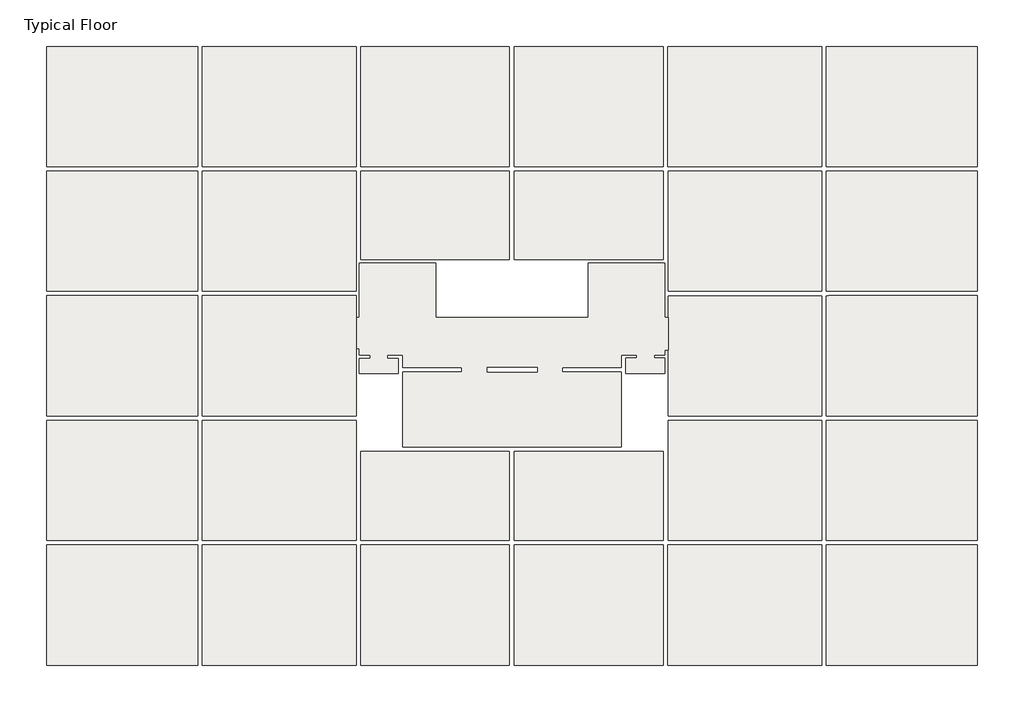
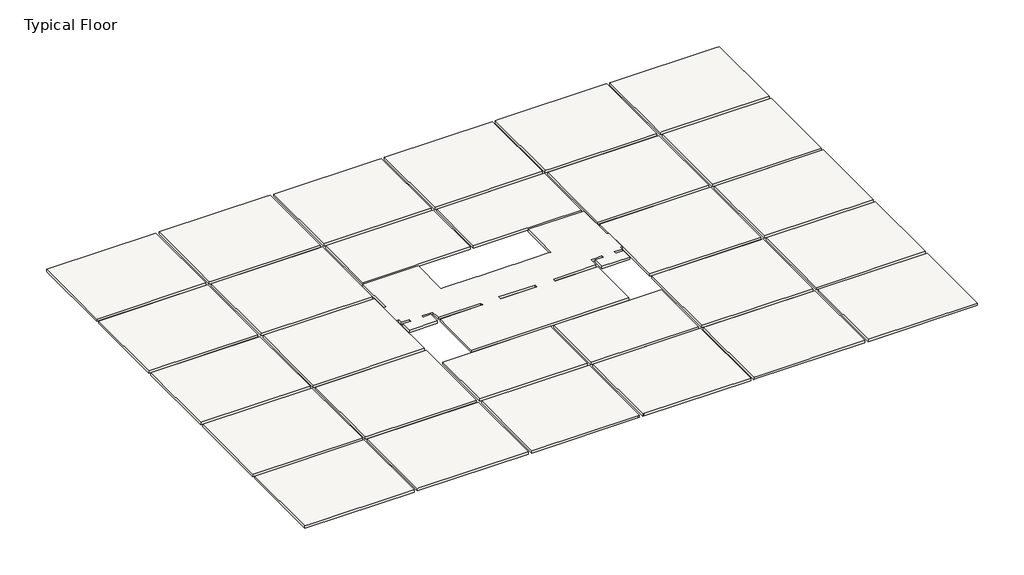
# One storey: 29 slabs.
"""IFC4 building model written with IfcOpenShell, lengths in millimetres."""

from ifc_helpers import new_model, si_unit, origin, place, context, project, spatial, faceted_brep, element, save

model = new_model("IFC4")

# Units and contexts
model_context = context("Model", 3, world=origin())
ifc_project = project(units=[si_unit("LENGTHUNIT", "METRE", prefix="MILLI")], contexts=[model_context])

# Site, building, storey
site = spatial("IfcSite", under=ifc_project)
building = spatial("IfcBuilding", under=site)
storey = spatial("IfcBuildingStorey", under=building, Name="Typical Floor", Elevation=3080.0)

# Slabs
placement = place(None, origin())
element("IfcSlab", 1, ObjectType="22", at=placement, inside=storey, context=model_context, shape_type="Brep", body=[
    faceted_brep([(-16600.7819865, 24775.4190544, 2860.0), (-16600.7819865, 17073.0342824, 2860.0), (-26299.1167382, 17073.0342824, 2860.0), (-26299.1167382, 24775.4190544, 2860.0), (-16600.7819865, 24775.4190544, 3080.0), (-16750.7819865, 24775.4190544, 3080.0), (-25999.1167382, 24775.4190544, 3080.0), (-26299.1167382, 24775.4190544, 3080.0), (-26299.1167382, 17073.0342824, 3080.0), (-16750.7819865, 17073.0342824, 3080.0), (-16600.7819865, 17073.0342824, 3080.0)], [[[0, 1, 2, 3]], [[4, 5, 6, 7, 8, 9, 10]], [[1, 0, 4, 10]], [[2, 1, 10, 9, 8]], [[3, 2, 8, 7]], [[0, 3, 7, 6, 5, 4]]]),
])
element("IfcSlab", 2, ObjectType="22", at=placement, inside=storey, context=model_context, shape_type="Brep", body=[
    faceted_brep([(-6447.328783, 24775.4190544, 2860.0), (-6447.328783, 17073.0342824, 2860.0), (-16300.7819865, 17073.0342824, 2860.0), (-16300.7819865, 24775.4190544, 2860.0), (-6447.328783, 24775.4190544, 3080.0), (-6747.328783, 24775.4190544, 3080.0), (-16150.7819865, 24775.4190544, 3080.0), (-16300.7819865, 24775.4190544, 3080.0), (-16300.7819865, 17073.0342824, 3080.0), (-16150.7819865, 17073.0342824, 3080.0), (-6747.328783, 17073.0342824, 3080.0), (-6447.328783, 17073.0342824, 3080.0)], [[[0, 1, 2, 3]], [[4, 5, 6, 7, 8, 9, 10, 11]], [[1, 0, 4, 11]], [[2, 1, 11, 10, 9, 8]], [[3, 2, 8, 7]], [[0, 3, 7, 6, 5, 4]]]),
])
element("IfcSlab", 3, ObjectType="22", at=placement, inside=storey, context=model_context, shape_type="Brep", body=[
    faceted_brep([(-6447.328783, 16773.0342824, 2860.0), (-6447.328783, 9078.7943074, 2860.0), (-16300.7819865, 9078.7943074, 2860.0), (-16300.7819865, 16773.0342824, 2860.0), (-6447.328783, 16773.0342824, 3080.0), (-6747.328783, 16773.0342824, 3080.0), (-16150.7819865, 16773.0342824, 3080.0), (-16300.7819865, 16773.0342824, 3080.0), (-16300.7819865, 9078.7943074, 3080.0), (-16150.7819865, 9078.7943074, 3080.0), (-6447.328783, 9078.7943074, 3080.0), (-6447.328783, 11089.5351037, 3080.0)], [[[0, 1, 2, 3]], [[4, 5, 6, 7, 8, 9, 10, 11]], [[1, 0, 4, 11, 10]], [[2, 1, 10, 9, 8]], [[3, 2, 8, 7]], [[0, 3, 7, 6, 5, 4]]]),
])
element("IfcSlab", 4, ObjectType="22", at=placement, inside=storey, context=model_context, shape_type="Brep", body=[
    faceted_brep([(-16600.7819865, 16773.0342824, 2860.0), (-16600.7819865, 9078.7943074, 2860.0), (-26299.1167382, 9078.7943074, 2860.0), (-26299.1167382, 16773.0342824, 2860.0), (-16600.7819865, 16773.0342824, 3080.0), (-16750.7819865, 16773.0342824, 3080.0), (-26299.1167382, 16773.0342824, 3080.0), (-26299.1167382, 9078.7943074, 3080.0), (-16750.7819865, 9078.7943074, 3080.0), (-16600.7819865, 9078.7943074, 3080.0)], [[[0, 1, 2, 3]], [[4, 5, 6, 7, 8, 9]], [[1, 0, 4, 9]], [[2, 1, 9, 8, 7]], [[3, 2, 7, 6]], [[0, 3, 6, 5, 4]]]),
])
element("IfcSlab", 5, ObjectType="22", at=placement, inside=storey, context=model_context, shape_type="Brep", body=[
    faceted_brep([(-16600.7819865, 8778.7943074, 2860.0), (-16600.7819865, 1074.102585, 2860.0), (-26299.1167382, 1074.102585, 2860.0), (-26299.1167382, 8778.7943074, 2860.0), (-16600.7819865, 8778.7943074, 3080.0), (-16750.7819865, 8778.7943074, 3080.0), (-26299.1167382, 8778.7943074, 3080.0), (-26299.1167382, 1074.102585, 3080.0), (-16750.7819865, 1074.102585, 3080.0), (-16600.7819865, 1074.102585, 3080.0)], [[[0, 1, 2, 3]], [[4, 5, 6, 7, 8, 9]], [[1, 0, 4, 9]], [[2, 1, 9, 8, 7]], [[3, 2, 7, 6]], [[0, 3, 6, 5, 4]]]),
])
element("IfcSlab", 6, ObjectType="22", at=placement, inside=storey, context=model_context, shape_type="Brep", body=[
    faceted_brep([(-16600.7819865, 774.102585, 2860.0), (-16600.7819865, -6920.4648963, 2860.0), (-26299.1167382, -6920.4648963, 2860.0), (-26299.1167382, 774.102585, 2860.0), (-16600.7819865, 774.102585, 3080.0), (-16750.7819865, 774.102585, 3080.0), (-26299.1167382, 774.102585, 3080.0), (-26299.1167382, -6920.4648963, 3080.0), (-16750.7819865, -6920.4648963, 3080.0), (-16600.7819865, -6920.4648963, 3080.0)], [[[0, 1, 2, 3]], [[4, 5, 6, 7, 8, 9]], [[1, 0, 4, 9]], [[2, 1, 9, 8, 7]], [[3, 2, 7, 6]], [[0, 3, 6, 5, 4]]]),
])
element("IfcSlab", 7, ObjectType="22", at=placement, inside=storey, context=model_context, shape_type="Brep", body=[
    faceted_brep([(-6447.328783, 774.102585, 2860.0), (-6447.328783, -6920.4648963, 2860.0), (-16300.7819865, -6920.4648963, 2860.0), (-16300.7819865, 774.102585, 2860.0), (-6447.328783, 774.102585, 3080.0), (-16150.7819865, 774.102585, 3080.0), (-16300.7819865, 774.102585, 3080.0), (-16300.7819865, -6920.4648963, 3080.0), (-16150.7819865, -6920.4648963, 3080.0), (-6747.328783, -6920.4648963, 3080.0), (-6447.328783, -6920.4648963, 3080.0), (-6447.328783, -1210.4648963, 3080.0)], [[[0, 1, 2, 3]], [[4, 5, 6, 7, 8, 9, 10, 11]], [[1, 0, 4, 11, 10]], [[2, 1, 10, 9, 8, 7]], [[3, 2, 7, 6]], [[0, 3, 6, 5, 4]]]),
])
element("IfcSlab", 8, ObjectType="22", at=placement, inside=storey, context=model_context, shape_type="Brep", body=[
    faceted_brep([(-16600.7819865, -7220.4648963, 2860.0), (-16600.7819865, -14918.7716477, 2860.0), (-26299.1167382, -14918.7716477, 2860.0), (-26299.1167382, -7220.4648963, 2860.0), (-16600.7819865, -7220.4648963, 3080.0), (-16750.7819865, -7220.4648963, 3080.0), (-26299.1167382, -7220.4648963, 3080.0), (-26299.1167382, -14918.7716477, 3080.0), (-25999.1167382, -14918.7716477, 3080.0), (-16750.7819865, -14918.7716477, 3080.0), (-16600.7819865, -14918.7716477, 3080.0)], [[[0, 1, 2, 3]], [[4, 5, 6, 7, 8, 9, 10]], [[1, 0, 4, 10]], [[2, 1, 10, 9, 8, 7]], [[3, 2, 7, 6]], [[0, 3, 6, 5, 4]]]),
])
element("IfcSlab", 9, ObjectType="22", at=placement, inside=storey, context=model_context, shape_type="Brep", body=[
    faceted_brep([(-6447.328783, -7220.4648963, 2860.0), (-6447.328783, -14918.7716477, 2860.0), (-16300.7819865, -14918.7716477, 2860.0), (-16300.7819865, -7220.4648963, 2860.0), (-6447.328783, -7220.4648963, 3080.0), (-6747.328783, -7220.4648963, 3080.0), (-16150.7819865, -7220.4648963, 3080.0), (-16300.7819865, -7220.4648963, 3080.0), (-16300.7819865, -14918.7716477, 3080.0), (-16150.7819865, -14918.7716477, 3080.0), (-6747.328783, -14918.7716477, 3080.0), (-6447.328783, -14918.7716477, 3080.0)], [[[0, 1, 2, 3]], [[4, 5, 6, 7, 8, 9, 10, 11]], [[1, 0, 4, 11]], [[2, 1, 11, 10, 9, 8]], [[3, 2, 8, 7]], [[0, 3, 7, 6, 5, 4]]]),
])
element("IfcSlab", 10, ObjectType="22", at=placement, inside=storey, context=model_context, shape_type="Brep", body=[
    faceted_brep([(3389.2018335, 24775.4190544, 2860.0), (3389.2018335, 17073.0342824, 2860.0), (-6147.328783, 17073.0342824, 2860.0), (-6147.328783, 24775.4190544, 2860.0), (3389.2018335, 24775.4190544, 3080.0), (3239.2018335, 24775.4190544, 3080.0), (-6147.328783, 24775.4190544, 3080.0), (-6147.328783, 17073.0342824, 3080.0), (3239.2018335, 17073.0342824, 3080.0), (3389.2018335, 17073.0342824, 3080.0)], [[[0, 1, 2, 3]], [[4, 5, 6, 7, 8, 9]], [[1, 0, 4, 9]], [[2, 1, 9, 8, 7]], [[3, 2, 7, 6]], [[0, 3, 6, 5, 4]]]),
])
element("IfcSlab", 11, ObjectType="22", at=placement, inside=storey, context=model_context, shape_type="Brep", body=[
    faceted_brep([(3389.2018335, 16773.0342824, 2860.0), (3389.2018335, 11089.5351037, 2860.0), (-6147.328783, 11089.5351037, 2860.0), (-6147.328783, 16773.0342824, 2860.0), (3389.2018335, 16773.0342824, 3080.0), (3239.2018335, 16773.0342824, 3080.0), (-6147.328783, 16773.0342824, 3080.0), (-6147.328783, 11089.5351037, 3080.0), (3389.2018335, 11089.5351037, 3080.0)], [[[0, 1, 2, 3]], [[4, 5, 6, 7, 8]], [[1, 0, 4, 8]], [[2, 1, 8, 7]], [[3, 2, 7, 6]], [[0, 3, 6, 5, 4]]]),
])
element("IfcSlab", 12, ObjectType="22", at=placement, inside=storey, context=model_context, shape_type="Brep", body=[
    faceted_brep([(-6147.328783, -14922.522162, 2860.0), (-6147.328783, -14918.7716477, 2860.0), (-6147.328783, -7220.4648963, 2860.0), (-6147.328783, -7220.13739, 2860.0), (3239.2018335, -7220.13739, 2860.0), (3239.2018335, -7220.4648963, 2860.0), (3389.2018335, -7220.4648963, 2860.0), (3389.2018335, -14918.7716477, 2860.0), (3239.2018335, -14918.7716477, 2860.0), (3239.2018335, -14922.522162, 2860.0), (-6147.328783, -7220.13739, 3080.0), (-6147.328783, -7220.4648963, 3080.0), (-6147.328783, -14918.7716477, 3080.0), (-6147.328783, -14922.522162, 3080.0), (3239.2018335, -14922.522162, 3080.0), (3239.2018335, -14918.7716477, 3080.0), (3389.2018335, -14918.7716477, 3080.0), (3389.2018335, -7220.4648963, 3080.0), (3239.2018335, -7220.4648963, 3080.0), (3239.2018335, -7220.13739, 3080.0)], [[[0, 1, 2, 3, 4, 5, 6, 7, 8, 9]], [[10, 11, 12, 13, 14, 15, 16, 17, 18, 19]], [[16, 7, 6, 17]], [[3, 10, 19, 4]], [[3, 2, 1, 0, 13, 12, 11, 10]], [[13, 0, 9, 14]], [[15, 8, 7, 16]], [[8, 15, 14, 9]], [[5, 18, 17, 6]], [[18, 5, 4, 19]]]),
])
element("IfcSlab", 13, ObjectType="22", at=placement, inside=storey, context=model_context, shape_type="Brep", body=[
    faceted_brep([(3389.2018335, -6920.4648963, 2860.0), (-6147.328783, -6920.4648963, 2860.0), (-6147.328783, -1210.4648963, 2860.0), (3389.2018335, -1210.4648963, 2860.0), (-6147.328783, -6920.4648963, 3080.0), (3239.2018335, -6920.4648963, 3080.0), (3389.2018335, -6920.4648963, 3080.0), (3389.2018335, -1210.4648963, 3080.0), (-3592.0160706, -1210.4648963, 3080.0), (-6147.328783, -1210.4648963, 3080.0)], [[[0, 1, 2, 3]], [[4, 5, 6, 7, 8, 9]], [[6, 0, 3, 7]], [[1, 4, 9, 2]], [[1, 0, 6, 5, 4]], [[2, 9, 8, 7, 3]]]),
])
element("IfcSlab", 14, ObjectType="22", at=placement, inside=storey, context=model_context, shape_type="Brep", body=[
    faceted_brep([(23700.3644839, 24775.4190544, 2860.0), (33398.6447783, 24775.4190544, 2860.0), (33398.6447783, 17073.0342824, 2860.0), (23700.3644839, 17073.0342824, 2860.0), (23700.3644839, 24775.4190544, 3080.0), (23700.3644839, 17073.0342824, 3080.0), (23850.3644839, 17073.0342824, 3080.0), (33398.6447783, 17073.0342824, 3080.0), (33398.6447783, 17222.0890048, 3080.0), (33398.6447783, 24775.4190544, 3080.0), (33098.6447783, 24775.4190544, 3080.0), (23850.3644839, 24775.4190544, 3080.0)], [[[0, 1, 2, 3]], [[4, 5, 6, 7, 8, 9, 10, 11]], [[0, 3, 5, 4]], [[3, 2, 7, 6, 5]], [[2, 1, 9, 8, 7]], [[1, 0, 4, 11, 10, 9]]]),
])
element("IfcSlab", 15, ObjectType="22", at=placement, inside=storey, context=model_context, shape_type="Brep", body=[
    faceted_brep([(13525.73245, 24775.4190544, 2860.0), (13557.9839294, 24775.4190544, 2860.0), (23400.3644839, 24775.4190544, 2860.0), (23400.3644839, 17073.0342824, 2860.0), (13557.9839294, 17073.0342824, 2860.0), (13525.73245, 17073.0342824, 2860.0), (13525.73245, 24775.4190544, 3080.0), (13525.73245, 17073.0342824, 3080.0), (13857.9839294, 17073.0342824, 3080.0), (23250.3644839, 17073.0342824, 3080.0), (23400.3644839, 17073.0342824, 3080.0), (23400.3644839, 24775.4190544, 3080.0), (23250.3644839, 24775.4190544, 3080.0), (13857.9839294, 24775.4190544, 3080.0)], [[[0, 1, 2, 3, 4, 5]], [[6, 7, 8, 9, 10, 11, 12, 13]], [[0, 5, 7, 6]], [[5, 4, 3, 10, 9, 8, 7]], [[3, 2, 11, 10]], [[2, 1, 0, 6, 13, 12, 11]]]),
])
element("IfcSlab", 16, ObjectType="22", at=placement, inside=storey, context=model_context, shape_type="Brep", body=[
    faceted_brep([(13557.9839294, 16773.0342824, 2860.0), (23400.3644839, 16773.0342824, 2860.0), (23400.3644839, 9072.0890048, 2860.0), (13557.9839294, 9072.0890048, 2860.0), (13557.9839294, 16773.0342824, 3080.0), (13557.9839294, 11089.5351037, 3080.0), (13557.9839294, 10889.5351037, 3080.0), (13557.9839294, 9072.0890048, 3080.0), (23250.3644839, 9072.0890048, 3080.0), (23400.3644839, 9072.0890048, 3080.0), (23400.3644839, 16773.0342824, 3080.0), (23250.3644839, 16773.0342824, 3080.0), (13857.9839294, 16773.0342824, 3080.0)], [[[0, 1, 2, 3]], [[4, 5, 6, 7, 8, 9, 10, 11, 12]], [[0, 3, 7, 6, 5, 4]], [[3, 2, 9, 8, 7]], [[2, 1, 10, 9]], [[1, 0, 4, 12, 11, 10]]]),
])
element("IfcSlab", 17, ObjectType="22", at=placement, inside=storey, context=model_context, shape_type="Brep", body=[
    faceted_brep([(23700.3644839, 16773.0342824, 2860.0), (33398.6447783, 16773.0342824, 2860.0), (33398.6447783, 9072.0890048, 2860.0), (23700.3644839, 9072.0890048, 2860.0), (23700.3644839, 16773.0342824, 3080.0), (23700.3644839, 9072.0890048, 3080.0), (23850.3644839, 9072.0890048, 3080.0), (33398.6447783, 9072.0890048, 3080.0), (33398.6447783, 9222.0890048, 3080.0), (33398.6447783, 16622.0890048, 3080.0), (33398.6447783, 16773.0342824, 3080.0), (23850.3644839, 16773.0342824, 3080.0)], [[[0, 1, 2, 3]], [[4, 5, 6, 7, 8, 9, 10, 11]], [[0, 3, 5, 4]], [[3, 2, 7, 6, 5]], [[2, 1, 10, 9, 8, 7]], [[1, 0, 4, 11, 10]]]),
])
element("IfcSlab", 18, ObjectType="22", at=placement, inside=storey, context=model_context, shape_type="Brep", body=[
    faceted_brep([(33398.6447783, 1074.102585, 2860.0), (23700.3644839, 1074.102585, 2860.0), (23700.3644839, 8772.0890048, 2860.0), (23850.3644839, 8772.0890048, 2860.0), (23850.3644839, 8778.7943074, 2860.0), (33398.6447783, 8778.7943074, 2860.0), (33398.6447783, 8772.0890048, 2860.0), (23700.3644839, 1074.102585, 3080.0), (23850.3644839, 1074.102585, 3080.0), (33398.6447783, 1074.102585, 3080.0), (33398.6447783, 1224.102585, 3080.0), (33398.6447783, 8622.0890048, 3080.0), (33398.6447783, 8778.7943074, 3080.0), (23850.3644839, 8778.7943074, 3080.0), (23850.3644839, 8772.0890048, 3080.0), (23700.3644839, 8772.0890048, 3080.0)], [[[0, 1, 2, 3, 4, 5, 6]], [[7, 8, 9, 10, 11, 12, 13, 14, 15]], [[1, 7, 15, 2]], [[1, 0, 9, 8, 7]], [[0, 6, 5, 12, 11, 10, 9]], [[12, 5, 4, 13]], [[14, 3, 2, 15]], [[3, 14, 13, 4]]]),
])
element("IfcSlab", 19, ObjectType="22", at=placement, inside=storey, context=model_context, shape_type="Brep", body=[
    faceted_brep([(23700.3644839, 774.102585, 2860.0), (33398.6447783, 774.102585, 2860.0), (33398.6447783, -6920.4648963, 2860.0), (23700.3644839, -6920.4648963, 2860.0), (23700.3644839, 774.102585, 3080.0), (23700.3644839, -6920.4648963, 3080.0), (23850.3644839, -6920.4648963, 3080.0), (33398.6447783, -6920.4648963, 3080.0), (33398.6447783, -6770.4648963, 3080.0), (33398.6447783, 624.102585, 3080.0), (33398.6447783, 774.102585, 3080.0), (23850.3644839, 774.102585, 3080.0)], [[[0, 1, 2, 3]], [[4, 5, 6, 7, 8, 9, 10, 11]], [[0, 3, 5, 4]], [[3, 2, 7, 6, 5]], [[2, 1, 10, 9, 8, 7]], [[1, 0, 4, 11, 10]]]),
])
element("IfcSlab", 20, ObjectType="22", at=placement, inside=storey, context=model_context, shape_type="Brep", body=[
    faceted_brep([(23700.3644839, -7220.4648963, 2860.0), (33398.6447783, -7220.4648963, 2860.0), (33398.6447783, -14918.7716477, 2860.0), (23700.3644839, -14918.7716477, 2860.0), (23700.3644839, -7220.4648963, 3080.0), (23700.3644839, -14918.7716477, 3080.0), (23850.3644839, -14918.7716477, 3080.0), (33098.6447783, -14918.7716477, 3080.0), (33398.6447783, -14918.7716477, 3080.0), (33398.6447783, -7370.4648963, 3080.0), (33398.6447783, -7220.4648963, 3080.0), (23850.3644839, -7220.4648963, 3080.0)], [[[0, 1, 2, 3]], [[4, 5, 6, 7, 8, 9, 10, 11]], [[0, 3, 5, 4]], [[3, 2, 8, 7, 6, 5]], [[2, 1, 10, 9, 8]], [[1, 0, 4, 11, 10]]]),
])
element("IfcSlab", 21, ObjectType="22", at=placement, inside=storey, context=model_context, shape_type="Brep", body=[
    faceted_brep([(13525.73245, -7220.4648963, 2860.0), (13557.9839294, -7220.4648963, 2860.0), (23400.3644839, -7220.4648963, 2860.0), (23400.3644839, -14918.7716477, 2860.0), (13557.9839294, -14918.7716477, 2860.0), (13525.73245, -14918.7716477, 2860.0), (13525.73245, -7220.4648963, 3080.0), (13525.73245, -14918.7716477, 3080.0), (13857.9839294, -14918.7716477, 3080.0), (23250.3644839, -14918.7716477, 3080.0), (23400.3644839, -14918.7716477, 3080.0), (23400.3644839, -7220.4648963, 3080.0), (23250.3644839, -7220.4648963, 3080.0), (13857.9839294, -7220.4648963, 3080.0)], [[[0, 1, 2, 3, 4, 5]], [[6, 7, 8, 9, 10, 11, 12, 13]], [[0, 5, 7, 6]], [[5, 4, 3, 10, 9, 8, 7]], [[3, 2, 11, 10]], [[2, 1, 0, 6, 13, 12, 11]]]),
])
element("IfcSlab", 22, ObjectType="22", at=placement, inside=storey, context=model_context, shape_type="Brep", body=[
    faceted_brep([(3689.2018335, 24775.4190544, 2860.0), (13257.9839294, 24775.4190544, 2860.0), (13257.9839294, 17073.0342824, 2860.0), (3689.2018335, 17073.0342824, 2860.0), (3689.2018335, 24775.4190544, 3080.0), (3689.2018335, 17073.0342824, 3080.0), (3839.2018335, 17073.0342824, 3080.0), (13257.9839294, 17073.0342824, 3080.0), (13257.9839294, 24775.4190544, 3080.0), (3839.2018335, 24775.4190544, 3080.0)], [[[0, 1, 2, 3]], [[4, 5, 6, 7, 8, 9]], [[0, 3, 5, 4]], [[3, 2, 7, 6, 5]], [[2, 1, 8, 7]], [[1, 0, 4, 9, 8]]]),
])
element("IfcSlab", 23, ObjectType="22", at=placement, inside=storey, context=model_context, shape_type="Brep", body=[
    faceted_brep([(3689.2018335, 16773.0342824, 2860.0), (13257.9839294, 16773.0342824, 2860.0), (13257.9839294, 11089.5351037, 2860.0), (3689.2018335, 11089.5351037, 2860.0), (3689.2018335, 16773.0342824, 3080.0), (3689.2018335, 11089.5351037, 3080.0), (13257.9839294, 11089.5351037, 3080.0), (13257.9839294, 16773.0342824, 3080.0), (3839.2018335, 16773.0342824, 3080.0)], [[[0, 1, 2, 3]], [[4, 5, 6, 7, 8]], [[0, 3, 5, 4]], [[3, 2, 6, 5]], [[2, 1, 7, 6]], [[1, 0, 4, 8, 7]]]),
])
element("IfcSlab", 24, ObjectType="22", at=placement, inside=storey, context=model_context, shape_type="Brep", body=[
    faceted_brep([(13257.9839294, -7220.13739, 2860.0), (13257.9839294, -7220.4648963, 2860.0), (13257.9839294, -14918.7716477, 2860.0), (13257.9839294, -14922.522162, 2860.0), (3839.2018335, -14922.522162, 2860.0), (3839.2018335, -14918.7716477, 2860.0), (3689.2018335, -14918.7716477, 2860.0), (3689.2018335, -7220.4648963, 2860.0), (3839.2018335, -7220.4648963, 2860.0), (3839.2018335, -7220.13739, 2860.0), (13257.9839294, -14922.522162, 3080.0), (13257.9839294, -14918.7716477, 3080.0), (13257.9839294, -7220.4648963, 3080.0), (13257.9839294, -7220.13739, 3080.0), (3839.2018335, -7220.13739, 3080.0), (3839.2018335, -7220.4648963, 3080.0), (3689.2018335, -7220.4648963, 3080.0), (3689.2018335, -14918.7716477, 3080.0), (3839.2018335, -14918.7716477, 3080.0), (3839.2018335, -14922.522162, 3080.0)], [[[0, 1, 2, 3, 4, 5, 6, 7, 8, 9]], [[10, 11, 12, 13, 14, 15, 16, 17, 18, 19]], [[6, 17, 16, 7]], [[13, 0, 9, 14]], [[3, 2, 1, 0, 13, 12, 11, 10]], [[3, 10, 19, 4]], [[5, 18, 17, 6]], [[18, 5, 4, 19]], [[8, 15, 14, 9]], [[15, 8, 7, 16]]]),
])
element("IfcSlab", 25, ObjectType="22", at=placement, inside=storey, context=model_context, shape_type="Brep", body=[
    faceted_brep([(3689.2018335, -6920.4648963, 2860.0), (3689.2018335, -1210.4648963, 2860.0), (13257.9839294, -1210.4648963, 2860.0), (13257.9839294, -6920.4648963, 2860.0), (3689.2018335, -6920.4648963, 3080.0), (3839.2018335, -6920.4648963, 3080.0), (13257.9839294, -6920.4648963, 3080.0), (13257.9839294, -1210.4648963, 3080.0), (10707.9839294, -1210.4648963, 3080.0), (3689.2018335, -1210.4648963, 3080.0)], [[[0, 1, 2, 3]], [[4, 5, 6, 7, 8, 9]], [[1, 0, 4, 9]], [[2, 1, 9, 8, 7]], [[3, 2, 7, 6]], [[0, 3, 6, 5, 4]]]),
])
element("IfcSlab", 26, ObjectType="22", at=placement, inside=storey, context=model_context, shape_type="Brep", body=[
    faceted_brep([(23400.3644839, 774.102585, 2860.0), (23400.3644839, -6920.4648963, 2860.0), (13557.9839294, -6920.4648963, 2860.0), (13557.9839294, 774.102585, 2860.0), (23400.3644839, 774.102585, 3080.0), (23250.3644839, 774.102585, 3080.0), (13557.9839294, 774.102585, 3080.0), (13557.9839294, -1210.4648963, 3080.0), (13557.9839294, -6920.4648963, 3080.0), (13857.9839294, -6920.4648963, 3080.0), (23250.3644839, -6920.4648963, 3080.0), (23400.3644839, -6920.4648963, 3080.0)], [[[0, 1, 2, 3]], [[4, 5, 6, 7, 8, 9, 10, 11]], [[1, 0, 4, 11]], [[2, 1, 11, 10, 9, 8]], [[3, 2, 8, 7, 6]], [[0, 3, 6, 5, 4]]]),
])
element("IfcSlab", 27, ObjectType="22", at=placement, inside=storey, context=model_context, shape_type="Brep", body=[
    faceted_brep([(-16300.7819865, 1074.102585, 2860.0), (-16300.7819865, 8778.7943074, 2860.0), (-6447.328783, 8778.7943074, 2860.0), (-6447.328783, 7389.5351037, 2860.0), (-6442.328783, 7389.5351037, 2860.0), (-6442.328783, 5389.5351037, 2860.0), (-6447.328783, 5389.5351037, 2860.0), (-6447.328783, 1074.102585, 2860.0), (-16300.7819865, 8778.7943074, 3080.0), (-16300.7819865, 1074.102585, 3080.0), (-16150.7819865, 1074.102585, 3080.0), (-6447.328783, 1074.102585, 3080.0), (-6447.328783, 5389.5351037, 3080.0), (-6442.328783, 5389.5351037, 3080.0), (-6442.328783, 7389.5351037, 3080.0), (-6447.328783, 7389.5351037, 3080.0), (-6447.328783, 8778.7943074, 3080.0), (-16150.7819865, 8778.7943074, 3080.0)], [[[0, 1, 2, 3, 4, 5, 6, 7]], [[8, 9, 10, 11, 12, 13, 14, 15, 16, 17]], [[13, 5, 4, 14]], [[9, 0, 7, 11, 10]], [[1, 0, 9, 8]], [[1, 8, 17, 16, 2]], [[6, 12, 11, 7]], [[12, 6, 5, 13]], [[15, 3, 2, 16]], [[3, 15, 14, 4]]]),
])
element("IfcSlab", 28, ObjectType="22", at=placement, inside=storey, context=model_context, shape_type="Brep", body=[
    faceted_brep([(13557.9839294, 8772.0890048, 2860.0), (23400.3644839, 8772.0890048, 2860.0), (23400.3644839, 1074.102585, 2860.0), (13557.9839294, 1074.102585, 2860.0), (13557.9839294, 5309.5351037, 2860.0), (13557.9839294, 7369.5351037, 2860.0), (13557.9839294, 8772.0890048, 3080.0), (13557.9839294, 7369.5351037, 3080.0), (13557.9839294, 5309.5351037, 3080.0), (13557.9839294, 1074.102585, 3080.0), (23250.3644839, 1074.102585, 3080.0), (23400.3644839, 1074.102585, 3080.0), (23400.3644839, 8772.0890048, 3080.0), (23250.3644839, 8772.0890048, 3080.0)], [[[0, 1, 2, 3, 4, 5]], [[6, 7, 8, 9, 10, 11, 12, 13]], [[1, 0, 6, 13, 12]], [[2, 1, 12, 11]], [[3, 2, 11, 10, 9]], [[0, 5, 4, 3, 9, 8, 7, 6]]]),
])
element("IfcSlab", 29, ObjectType="22", at=placement, inside=storey, context=model_context, shape_type="Brep", body=[
    faceted_brep([(13357.9839294, 5309.5351037, 2860.0), (13357.9839294, 4977.6133465, 2860.0), (12657.9839294, 4977.6133465, 2860.0), (12657.9839294, 4777.6133465, 2860.0), (13357.9839294, 4777.6133465, 2860.0), (13357.9839294, 3778.9683527, 2860.0), (10857.9839294, 3778.9683527, 2860.0), (10857.9839294, 3877.6133465, 2860.0), (10857.9839294, 4177.6133465, 2860.0), (10857.9839294, 4777.6133465, 2860.0), (11557.9839294, 4777.6133465, 2860.0), (11557.9839294, 4977.6133465, 2860.0), (10857.9839294, 4977.6133465, 2860.0), (10557.9839294, 4977.6133465, 2860.0), (10557.9839294, 4177.6133465, 2860.0), (6757.9839294, 4177.6133465, 2860.0), (6757.9839294, 3877.6133465, 2860.0), (10557.9839294, 3877.6133465, 2860.0), (10557.9839294, -910.4648963, 2860.0), (-3442.0160706, -910.4648963, 2860.0), (-3442.0160706, 3877.6133465, 2860.0), (337.9839294, 3877.6133465, 2860.0), (337.9839294, 4177.6133465, 2860.0), (-3442.0160706, 4177.6133465, 2860.0), (-3442.0160706, 4969.5351037, 2860.0), (-3742.0160706, 4969.5351037, 2860.0), (-4442.0160706, 4969.5351037, 2860.0), (-4442.0160706, 4769.5351037, 2860.0), (-3742.0160706, 4769.5351037, 2860.0), (-3742.0160706, 3781.3337247, 2860.0), (-6247.328783, 3781.3337247, 2860.0), (-6247.328783, 4769.5351037, 2860.0), (-5542.0160706, 4769.5351037, 2860.0), (-5542.0160706, 4969.5351037, 2860.0), (-6247.328783, 4969.5351037, 2860.0), (-6247.328783, 5389.5351037, 2860.0), (-6442.328783, 5389.5351037, 2860.0), (-6442.328783, 7389.5351037, 2860.0), (-6247.328783, 7389.5351037, 2860.0), (-6247.328783, 10889.5351037, 2860.0), (-1346.9159577, 10889.5351037, 2860.0), (-1346.9159577, 7369.5351037, 2860.0), (-1146.9159577, 7369.5351037, 2860.0), (1839.2018335, 7369.5351037, 2860.0), (2039.2018335, 7369.5351037, 2860.0), (5039.2018335, 7369.5351037, 2860.0), (5239.2018335, 7369.5351037, 2860.0), (8239.2018335, 7369.5351037, 2860.0), (8439.2018335, 7369.5351037, 2860.0), (8439.2018335, 10889.5351037, 2860.0), (13357.9839294, 10889.5351037, 2860.0), (13357.9839294, 7369.5351037, 2860.0), (13557.9839294, 7369.5351037, 2860.0), (13557.9839294, 5309.5351037, 2860.0), (5157.9839294, 4177.6133465, 2860.0), (1957.9839294, 4177.6133465, 2860.0), (1957.9839294, 3877.6133465, 2860.0), (5157.9839294, 3877.6133465, 2860.0), (13357.9839294, 4977.6133465, 3080.0), (13357.9839294, 5309.5351037, 3080.0), (13557.9839294, 5309.5351037, 3080.0), (13557.9839294, 7369.5351037, 3080.0), (13357.9839294, 7369.5351037, 3080.0), (13357.9839294, 10889.5351037, 3080.0), (8439.2018335, 10889.5351037, 3080.0), (8439.2018335, 7369.5351037, 3080.0), (8239.2018335, 7369.5351037, 3080.0), (5239.2018335, 7369.5351037, 3080.0), (5039.2018335, 7369.5351037, 3080.0), (2039.2018335, 7369.5351037, 3080.0), (1839.2018335, 7369.5351037, 3080.0), (-1146.9159577, 7369.5351037, 3080.0), (-1346.9159577, 7369.5351037, 3080.0), (-1346.9159577, 10889.5351037, 3080.0), (-6247.328783, 10889.5351037, 3080.0), (-6247.328783, 7389.5351037, 3080.0), (-6442.328783, 7389.5351037, 3080.0), (-6442.328783, 5389.5351037, 3080.0), (-6247.328783, 5389.5351037, 3080.0), (-6247.328783, 4969.5351037, 3080.0), (-5542.0160706, 4969.5351037, 3080.0), (-5542.0160706, 4769.5351037, 3080.0), (-6247.328783, 4769.5351037, 3080.0), (-6247.328783, 3781.3337247, 3080.0), (-3742.0160706, 3781.3337247, 3080.0), (-3742.0160706, 4769.5351037, 3080.0), (-4442.0160706, 4769.5351037, 3080.0), (-4442.0160706, 4969.5351037, 3080.0), (-3742.0160706, 4969.5351037, 3080.0), (-3442.0160706, 4969.5351037, 3080.0), (-3442.0160706, 4177.6133465, 3080.0), (337.9839294, 4177.6133465, 3080.0), (337.9839294, 3877.6133465, 3080.0), (-3442.0160706, 3877.6133465, 3080.0), (-3442.0160706, -910.4648963, 3080.0), (10557.9839294, -910.4648963, 3080.0), (10557.9839294, 3877.6133465, 3080.0), (6757.9839294, 3877.6133465, 3080.0), (6757.9839294, 4177.6133465, 3080.0), (10557.9839294, 4177.6133465, 3080.0), (10557.9839294, 4977.6133465, 3080.0), (10857.9839294, 4977.6133465, 3080.0), (11557.9839294, 4977.6133465, 3080.0), (11557.9839294, 4777.6133465, 3080.0), (10857.9839294, 4777.6133465, 3080.0), (10857.9839294, 4177.6133465, 3080.0), (10857.9839294, 3877.6133465, 3080.0), (10857.9839294, 3778.9683527, 3080.0), (13357.9839294, 3778.9683527, 3080.0), (13357.9839294, 4777.6133465, 3080.0), (12657.9839294, 4777.6133465, 3080.0), (12657.9839294, 4977.6133465, 3080.0), (1957.9839294, 4177.6133465, 3080.0), (5157.9839294, 4177.6133465, 3080.0), (5157.9839294, 3877.6133465, 3080.0), (1957.9839294, 3877.6133465, 3080.0)], [[[0, 1, 2, 3, 4, 5, 6, 7, 8, 9, 10, 11, 12, 13, 14, 15, 16, 17, 18, 19, 20, 21, 22, 23, 24, 25, 26, 27, 28, 29, 30, 31, 32, 33, 34, 35, 36, 37, 38, 39, 40, 41, 42, 43, 44, 45, 46, 47, 48, 49, 50, 51, 52, 53], [54, 55, 56, 57]], [[58, 59, 60, 61, 62, 63, 64, 65, 66, 67, 68, 69, 70, 71, 72, 73, 74, 75, 76, 77, 78, 79, 80, 81, 82, 83, 84, 85, 86, 87, 88, 89, 90, 91, 92, 93, 94, 95, 96, 97, 98, 99, 100, 101, 102, 103, 104, 105, 106, 107, 108, 109, 110, 111], [112, 113, 114, 115]], [[1, 0, 59, 58]], [[2, 1, 58, 111]], [[3, 2, 111, 110]], [[4, 3, 110, 109]], [[5, 4, 109, 108]], [[6, 5, 108, 107]], [[6, 107, 106, 105, 104, 9, 8, 7]], [[10, 9, 104, 103]], [[11, 10, 103, 102]], [[11, 102, 101, 100, 13, 12]], [[14, 13, 100, 99]], [[15, 14, 99, 98]], [[16, 15, 98, 97]], [[17, 16, 97, 96]], [[18, 17, 96, 95]], [[19, 18, 95, 94]], [[20, 19, 94, 93]], [[21, 20, 93, 92]], [[22, 21, 92, 91]], [[23, 22, 91, 90]], [[24, 23, 90, 89]], [[24, 89, 88, 87, 26, 25]], [[27, 26, 87, 86]], [[28, 27, 86, 85]], [[29, 28, 85, 84]], [[30, 29, 84, 83]], [[31, 30, 83, 82]], [[32, 31, 82, 81]], [[33, 32, 81, 80]], [[34, 33, 80, 79]], [[35, 34, 79, 78]], [[35, 78, 77, 36]], [[75, 38, 37, 76]], [[39, 38, 75, 74]], [[40, 39, 74, 73]], [[41, 40, 73, 72]], [[41, 72, 71, 70, 69, 68, 67, 66, 65, 48, 47, 46, 45, 44, 43, 42]], [[49, 48, 65, 64]], [[50, 49, 64, 63]], [[51, 50, 63, 62]], [[52, 51, 62, 61]], [[53, 52, 61, 60]], [[0, 53, 60, 59]], [[55, 54, 113, 112]], [[56, 55, 112, 115]], [[57, 56, 115, 114]], [[54, 57, 114, 113]], [[37, 36, 77, 76]]]),
])

save(model, "model.ifc")

# Revit data of these elements
# Type "22"
#   Function = 0
#   Layers, outside or top first: 22 cm "Concrete" (function 1)
# Element 1 (IfcSlab, "22")
#   Mark = "S1"
#   SOFiSTiK_AMG_Comments = ""
#   Height Offset From Level = 0 cm
#   built-in parameter 1001954 = 1
#   SOFiSTiK_AMG_Scheduled = yes
#   SOFiSTiK_AMG_Adjusted = yes
#   Phase Created = New Construction
#   Materials on its faces: "Concrete"
# Element 2 (IfcSlab, "22")
#   Mark = "S2"
#   SOFiSTiK_AMG_Comments = ""
#   Height Offset From Level = 0 cm
#   built-in parameter 1001954 = 1
#   SOFiSTiK_AMG_Scheduled = yes
#   SOFiSTiK_AMG_Adjusted = yes
#   Phase Created = New Construction
#   Materials on its faces: "Concrete"
# Element 3 (IfcSlab, "22")
#   Mark = "S3"
#   SOFiSTiK_AMG_Comments = ""
#   Height Offset From Level = 0 cm
#   built-in parameter 1001954 = 1
#   SOFiSTiK_AMG_Scheduled = yes
#   SOFiSTiK_AMG_Adjusted = yes
#   Phase Created = New Construction
#   Materials on its faces: "Concrete"
# Element 4 (IfcSlab, "22")
#   Mark = "S4"
#   SOFiSTiK_AMG_Comments = ""
#   Height Offset From Level = 0 cm
#   built-in parameter 1001954 = 1
#   SOFiSTiK_AMG_Scheduled = yes
#   SOFiSTiK_AMG_Adjusted = yes
#   Phase Created = New Construction
#   Materials on its faces: "Concrete"
# Element 5 (IfcSlab, "22")
#   Mark = "S5"
#   SOFiSTiK_AMG_Comments = ""
#   Height Offset From Level = 0 cm
#   built-in parameter 1001954 = 1
#   SOFiSTiK_AMG_Scheduled = yes
#   SOFiSTiK_AMG_Adjusted = yes
#   Phase Created = New Construction
#   Materials on its faces: "Concrete"
# Element 6 (IfcSlab, "22")
#   Mark = "S6"
#   SOFiSTiK_AMG_Comments = ""
#   Height Offset From Level = 0 cm
#   built-in parameter 1001954 = 1
#   SOFiSTiK_AMG_Scheduled = yes
#   SOFiSTiK_AMG_Adjusted = yes
#   Phase Created = New Construction
#   Materials on its faces: "Concrete"
# Element 7 (IfcSlab, "22")
#   Mark = "S7"
#   SOFiSTiK_AMG_Comments = ""
#   Height Offset From Level = 0 cm
#   built-in parameter 1001954 = 1
#   SOFiSTiK_AMG_Scheduled = yes
#   SOFiSTiK_AMG_Adjusted = yes
#   Phase Created = New Construction
#   Materials on its faces: "Concrete"
# Element 8 (IfcSlab, "22")
#   Mark = "S8"
#   SOFiSTiK_AMG_Comments = ""
#   Height Offset From Level = 0 cm
#   built-in parameter 1001954 = 1
#   SOFiSTiK_AMG_Scheduled = yes
#   SOFiSTiK_AMG_Adjusted = yes
#   Phase Created = New Construction
#   Materials on its faces: "Concrete"
# Element 9 (IfcSlab, "22")
#   Mark = "S9"
#   SOFiSTiK_AMG_Comments = ""
#   Height Offset From Level = 0 cm
#   built-in parameter 1001954 = 1
#   SOFiSTiK_AMG_Scheduled = yes
#   SOFiSTiK_AMG_Adjusted = yes
#   Phase Created = New Construction
#   Materials on its faces: "Concrete"
# Element 10 (IfcSlab, "22")
#   Mark = "S10"
#   SOFiSTiK_AMG_Comments = ""
#   Height Offset From Level = 0 cm
#   built-in parameter 1001954 = 1
#   SOFiSTiK_AMG_Scheduled = yes
#   SOFiSTiK_AMG_Adjusted = yes
#   Phase Created = New Construction
#   Materials on its faces: "Concrete"
# Element 11 (IfcSlab, "22")
#   Mark = "S11"
#   SOFiSTiK_AMG_Comments = ""
#   Height Offset From Level = 0 cm
#   built-in parameter 1001954 = 1
#   SOFiSTiK_AMG_Scheduled = yes
#   SOFiSTiK_AMG_Adjusted = yes
#   Phase Created = New Construction
#   Materials on its faces: "Concrete"
# Element 12 (IfcSlab, "22")
#   Mark = "S12"
#   SOFiSTiK_AMG_Comments = ""
#   Height Offset From Level = 0 cm
#   built-in parameter 1001954 = 1
#   SOFiSTiK_AMG_Scheduled = yes
#   SOFiSTiK_AMG_Adjusted = yes
#   Phase Created = New Construction
#   Materials on its faces: "Concrete"
# Element 13 (IfcSlab, "22")
#   Mark = "S13"
#   SOFiSTiK_AMG_Comments = ""
#   Height Offset From Level = 0 cm
#   built-in parameter 1001954 = 1
#   SOFiSTiK_AMG_Scheduled = yes
#   SOFiSTiK_AMG_Adjusted = yes
#   Phase Created = New Construction
#   Materials on its faces: "Concrete"
# Element 14 (IfcSlab, "22")
#   Mark = "S14"
#   SOFiSTiK_AMG_Comments = ""
#   built-in parameter 1001955 = 3.14159 (stored number, unit not read)
#   Height Offset From Level = 0 cm
#   built-in parameter 1001954 = 1
#   SOFiSTiK_AMG_Scheduled = yes
#   SOFiSTiK_AMG_Adjusted = yes
#   Phase Created = New Construction
#   Materials on its faces: "Concrete"
# Element 15 (IfcSlab, "22")
#   Mark = "S15"
#   SOFiSTiK_AMG_Comments = ""
#   built-in parameter 1001955 = 3.14159 (stored number, unit not read)
#   Height Offset From Level = 0 cm
#   built-in parameter 1001954 = 1
#   SOFiSTiK_AMG_Scheduled = yes
#   SOFiSTiK_AMG_Adjusted = yes
#   Phase Created = New Construction
#   Materials on its faces: "Concrete"
# Element 16 (IfcSlab, "22")
#   Mark = "S16"
#   SOFiSTiK_AMG_Comments = ""
#   built-in parameter 1001955 = 3.14159 (stored number, unit not read)
#   Height Offset From Level = 0 cm
#   built-in parameter 1001954 = 1
#   SOFiSTiK_AMG_Scheduled = yes
#   SOFiSTiK_AMG_Adjusted = yes
#   Phase Created = New Construction
#   Materials on its faces: "Concrete"
# Element 17 (IfcSlab, "22")
#   Mark = "S17"
#   SOFiSTiK_AMG_Comments = ""
#   built-in parameter 1001955 = 3.14159 (stored number, unit not read)
#   Height Offset From Level = 0 cm
#   built-in parameter 1001954 = 1
#   SOFiSTiK_AMG_Scheduled = yes
#   SOFiSTiK_AMG_Adjusted = yes
#   Phase Created = New Construction
#   Materials on its faces: "Concrete"
# Element 18 (IfcSlab, "22")
#   Mark = "S18"
#   SOFiSTiK_AMG_Comments = ""
#   built-in parameter 1001955 = 3.14159 (stored number, unit not read)
#   Height Offset From Level = 0 cm
#   built-in parameter 1001954 = 1
#   SOFiSTiK_AMG_Scheduled = yes
#   SOFiSTiK_AMG_Adjusted = yes
#   Phase Created = New Construction
#   Materials on its faces: "Concrete"
# Element 19 (IfcSlab, "22")
#   Mark = "S19"
#   SOFiSTiK_AMG_Comments = ""
#   built-in parameter 1001955 = 3.14159 (stored number, unit not read)
#   Height Offset From Level = 0 cm
#   built-in parameter 1001954 = 1
#   SOFiSTiK_AMG_Scheduled = yes
#   SOFiSTiK_AMG_Adjusted = yes
#   Phase Created = New Construction
#   Materials on its faces: "Concrete"
# Element 20 (IfcSlab, "22")
#   Mark = "S20"
#   SOFiSTiK_AMG_Comments = ""
#   built-in parameter 1001955 = 3.14159 (stored number, unit not read)
#   Height Offset From Level = 0 cm
#   built-in parameter 1001954 = 1
#   SOFiSTiK_AMG_Scheduled = yes
#   SOFiSTiK_AMG_Adjusted = yes
#   Phase Created = New Construction
#   Materials on its faces: "Concrete"
# Element 21 (IfcSlab, "22")
#   Mark = "S21"
#   SOFiSTiK_AMG_Comments = ""
#   built-in parameter 1001955 = 3.14159 (stored number, unit not read)
#   Height Offset From Level = 0 cm
#   built-in parameter 1001954 = 1
#   SOFiSTiK_AMG_Scheduled = yes
#   SOFiSTiK_AMG_Adjusted = yes
#   Phase Created = New Construction
#   Materials on its faces: "Concrete"
# Element 22 (IfcSlab, "22")
#   Mark = "S22"
#   SOFiSTiK_AMG_Comments = ""
#   built-in parameter 1001955 = 3.14159 (stored number, unit not read)
#   Height Offset From Level = 0 cm
#   built-in parameter 1001954 = 1
#   SOFiSTiK_AMG_Scheduled = yes
#   SOFiSTiK_AMG_Adjusted = yes
#   Phase Created = New Construction
#   Materials on its faces: "Concrete"
# Element 23 (IfcSlab, "22")
#   Mark = "S23"
#   SOFiSTiK_AMG_Comments = ""
#   built-in parameter 1001955 = 3.14159 (stored number, unit not read)
#   Height Offset From Level = 0 cm
#   built-in parameter 1001954 = 1
#   SOFiSTiK_AMG_Scheduled = yes
#   SOFiSTiK_AMG_Adjusted = yes
#   Phase Created = New Construction
#   Materials on its faces: "Concrete"
# Element 24 (IfcSlab, "22")
#   Mark = "S24"
#   SOFiSTiK_AMG_Comments = ""
#   built-in parameter 1001955 = 3.14159 (stored number, unit not read)
#   Height Offset From Level = 0 cm
#   built-in parameter 1001954 = 1
#   SOFiSTiK_AMG_Scheduled = yes
#   SOFiSTiK_AMG_Adjusted = yes
#   Phase Created = New Construction
#   Materials on its faces: "Concrete"
# Element 25 (IfcSlab, "22")
#   Mark = "S25"
#   SOFiSTiK_AMG_Comments = ""
#   built-in parameter 1001955 = 3.14159 (stored number, unit not read)
#   Height Offset From Level = 0 cm
#   built-in parameter 1001954 = 1
#   SOFiSTiK_AMG_Scheduled = yes
#   SOFiSTiK_AMG_Adjusted = yes
#   Phase Created = New Construction
#   Materials on its faces: "Concrete"
# Element 26 (IfcSlab, "22")
#   Mark = "S26"
#   SOFiSTiK_AMG_Comments = ""
#   Height Offset From Level = 0 cm
#   built-in parameter 1001954 = 1
#   SOFiSTiK_AMG_Scheduled = yes
#   SOFiSTiK_AMG_Adjusted = yes
#   Phase Created = New Construction
#   Materials on its faces: "Concrete"
# Element 27 (IfcSlab, "22")
#   Mark = "S27"
#   SOFiSTiK_AMG_Comments = ""
#   Height Offset From Level = 0 cm
#   built-in parameter 1001954 = 1
#   SOFiSTiK_AMG_Scheduled = yes
#   SOFiSTiK_AMG_Adjusted = yes
#   Phase Created = New Construction
#   Materials on its faces: "Concrete"
# Element 28 (IfcSlab, "22")
#   Mark = "S28"
#   SOFiSTiK_AMG_Comments = ""
#   built-in parameter 1001955 = 3.14159 (stored number, unit not read)
#   Height Offset From Level = 0 cm
#   built-in parameter 1001954 = 1
#   SOFiSTiK_AMG_Scheduled = yes
#   SOFiSTiK_AMG_Adjusted = yes
#   Phase Created = New Construction
#   Materials on its faces: "Concrete"
# Element 29 (IfcSlab, "22")
#   Mark = "S29"
#   SOFiSTiK_AMG_Comments = ""
#   built-in parameter 1001955 = 3.14159 (stored number, unit not read)
#   Height Offset From Level = 0 cm
#   built-in parameter 1001954 = 1
#   SOFiSTiK_AMG_Scheduled = yes
#   SOFiSTiK_AMG_Adjusted = yes
#   Phase Created = New Construction
#   Materials on its faces: "Concrete"
# Materials
#   "Concrete": class "Concrete", colour RGB 192 192 192, transparency 0, Keynote = "01000", Description = "Cast-in-place concrete", Cost = 0
